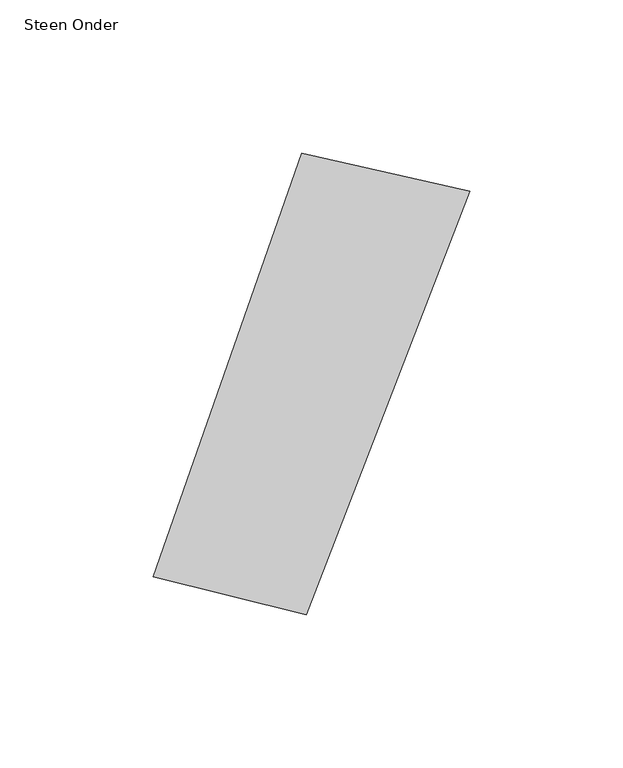
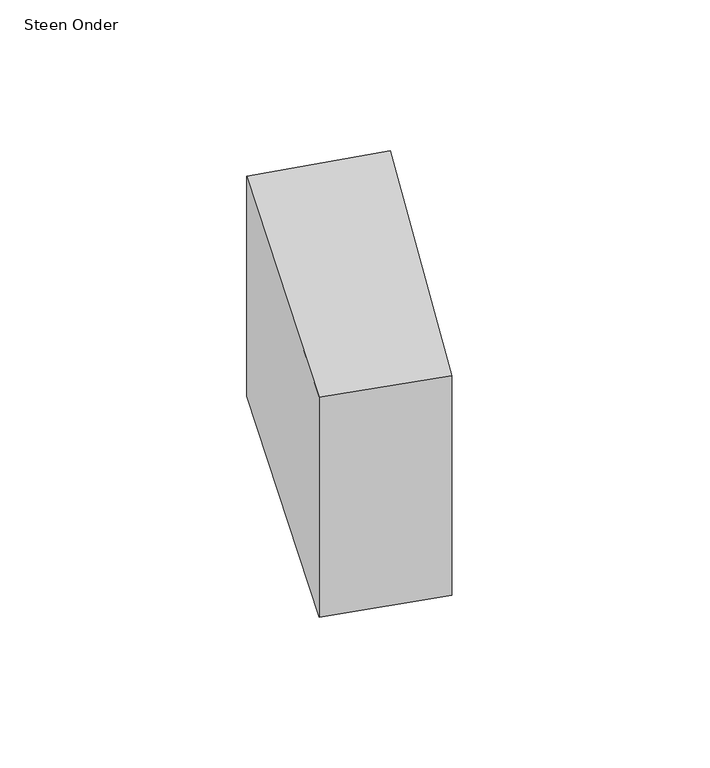
"""IFC4 building model written with IfcOpenShell, lengths in millimetres: proxy geometry, 00_GMA_steen_versie_4 : Steen Onder."""

from ifc_helpers import new_model, si_unit, origin, origin_with_axes, place, context, project, spatial, polyline, outline, extrude, source, transform, mapped, element, save


def steen_onder_81eb11de(model_context):
    return source(origin(), model_context, "Body", "SweptSolid", [
        extrude(outline(polyline([(126.404272, 136.4021132), (73.1966298, -1.4709909), (23.4060832, 10.85532), (71.7350528, 148.7786201), (126.404272, 136.4021132)])), origin_with_axes(), (0.0, 0.0, 1.0), 100.0),
    ])


if __name__ == "__main__":
    model = new_model("IFC4")
    model_context = context("Model", 3, world=origin())
    ifc_project = project(units=[si_unit("LENGTHUNIT", "METRE", prefix="MILLI")], contexts=[model_context])
    site = spatial("IfcSite", under=ifc_project)
    building = spatial("IfcBuilding", under=site)
    placement = place(None, origin())
    steen_onder_shape = steen_onder_81eb11de(model_context)
    element("IfcBuildingElementProxy", 1, Name="00_GMA_steen_versie_4 : Steen Onder", ObjectType="00_GMA_steen_versie_4 : Steen Onder", at=placement, inside=building, context=model_context, shape_type="MappedRepresentation", body=[
        mapped(steen_onder_shape, transform((0.0, 0.0, 0.0), x_axis=(1.0, 0.0, 0.0), y_axis=(0.0, 1.0, 0.0), z_axis=(0.0, 0.0, 1.0))),
    ])
    save(model, "model.ifc")

# Revit data of these elements
# Type "00_GMA_steen_versie_4 : Steen Onder"
#   StootVoegHalfBoven [instance default] = 5 mm
#   StootVoegHalf [instance default] = 5 mm
#   StootVoegBreedteOnder = 10 mm
#   StootVoegBreedteBoven = 10 mm
#   Steendikte = 100 mm
#   LintVoegOnderHalf = 0 mm
#   LintVoegOnder = 0 mm
#   LintVoegBovenHalf = 5 mm
#   LintVoegBoven = 10 mm
#   materiaal = none
#   MateriaalVoeg = none
#   Default Elevation = 0
